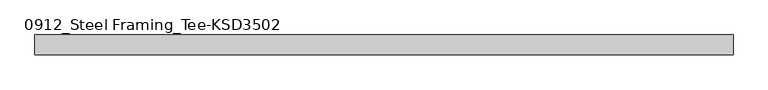
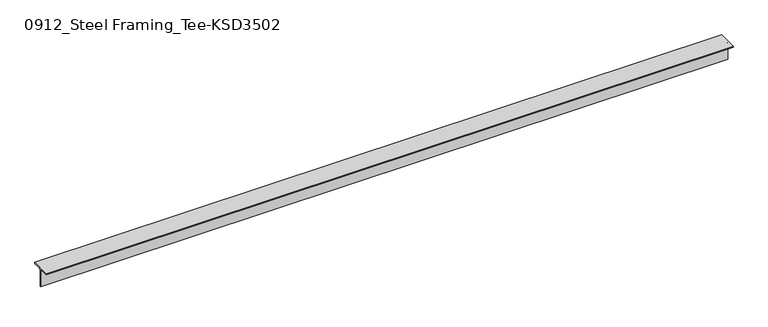
"""IFC4 building model written with IfcOpenShell, lengths in millimetres: member geometry, 0912_Steel Framing_Tee-KSD3502 : H_SB_ASB_CT-150x150x6.5x9."""

from ifc_helpers import new_model, si_unit, point, frame, frame_2d, origin, place, context, project, spatial, polyline, circle_curve, trimmed, segment, composite_curve, outline, extrude, source, transform, mapped, element, save


def member_0912_steel_framing_tee_ksd3502_229a0811(model_context):
    return source(origin(), model_context, "Body", "SweptSolid", [
        extrude(outline(composite_curve([segment(polyline([(-75.0, 75.0), (75.0, 75.0), (75.0, 66.0), (16.25, 66.0)]), True, "CONTINUOUS"), segment(trimmed(circle_curve(frame_2d((16.25, 53.0)), 13.0), [point((16.25, 66.0))], [point((3.25, 53.0))], True, "CARTESIAN"), True, "CONTINUOUS"), segment(polyline([(3.25, 53.0), (3.25, -75.0), (-3.25, -75.0), (-3.25, 53.0)]), True, "CONTINUOUS"), segment(trimmed(circle_curve(frame_2d((-16.25, 53.0)), 13.0), [point((-3.25, 53.0))], [point((-16.25, 66.0))], True, "CARTESIAN"), True, "CONTINUOUS"), segment(polyline([(-16.25, 66.0), (-75.0, 66.0), (-75.0, 75.0)]), True, "CONTINUOUS")], self_intersect=False)), frame((-2735.35, 0.0, 0.0), z_axis=(1.0, 0.0, 0.0), x_axis=(0.0, 1.0, 0.0)), (0.0, 0.0, 1.0), 5312.4),
    ])


if __name__ == "__main__":
    model = new_model("IFC4")
    model_context = context("Model", 3, world=origin())
    ifc_project = project(units=[si_unit("LENGTHUNIT", "METRE", prefix="MILLI")], contexts=[model_context])
    site = spatial("IfcSite", under=ifc_project)
    building = spatial("IfcBuilding", under=site)
    placement = place(None, origin())
    member_0912_steel_framing_tee_ksd3502_shape = member_0912_steel_framing_tee_ksd3502_229a0811(model_context)
    element("IfcMember", 1, ObjectType="0912_Steel Framing_Tee-KSD3502 : H_SB_ASB_CT-150x150x6.5x9", at=placement, inside=building, context=model_context, shape_type="MappedRepresentation", body=[
        mapped(member_0912_steel_framing_tee_ksd3502_shape, transform((0.0, 0.0, 0.0), x_axis=(1.0, 0.0, 0.0), y_axis=(0.0, 1.0, 0.0), z_axis=(0.0, 0.0, 1.0))),
    ])
    save(model, "model.ifc")

# Revit data of these elements
# Type "0912_Steel Framing_Tee-KSD3502 : H_SB_ASB_CT-150x150x6.5x9"
#   H_WM Code_1 = "S01AA003-00001 | Main Steel Structure Fabrication Work | Shelter/Building | Light Steel - Standard (30KG/M>Weight) | Material: (   )"
#   H_WM Code_2 = "S03AA029-00001 | Main Steel Structure Erection Work | Shelter/Building | Light Steel (30KG/M>Weight) | Material: (   )"
#   H_WM Code_3 = "S01AA010-00001 | Main Steel Structure Fabrication Work | Shelter/Building | Steel Painting/Coating | for Non-Fireproofed Steel Surface, Surface Preparation, Primer, Second & Final Coat | Material: (   )"
#   H_Q'ty Cal Type Tag = "SB-Q2"
#   Width = 15.0 cm
#   Web Thickness = 0.65 cm
#   Web Fillet = 1.3 cm
#   Section Area = 23.39 cm²
#   Perimeter = 0.60 m²/m
#   Nominal Weight = 18.40 kgf/m
#   Height = 15.0 cm
#   Flange Thickness = 0.9 cm
#   Centroid Vertical = 7.5 cm
#   Centroid Horizontal = 7.5 cm
#   Length [instance default] = 1.5000 m
#   Structural Material [instance default] = Steel, 45-345
#   Warping Constant = (empty or 0)
#   Torsional Moment of Inertia = 0
#   Section Name Key = ""
#   Plastic Modulus weak axis = 0
#   Plastic Modulus strong axis = 0
#   Moment of Inertia weak axis = 0
#   Moment of Inertia strong axis = 0
#   Elastic Modulus weak axis = 0
#   Elastic Modulus strong axis = 0
#   Bolt Spacing = 0
#   Assembly Code = ""
# Element 1 (IfcMember, "0912_Steel Framing_Tee-KSD3502 : H_SB_ASB_CT-150x150x6.5x9")
#   Structural Material = none
# Materials
#   "Steel, 45-345": class "Metal", colour RGB 189 187 185, transparency 0, Description = "Steel 345 MPa", Cost = 0
